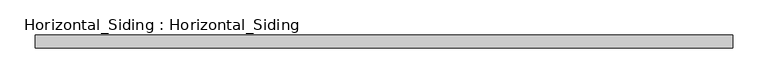
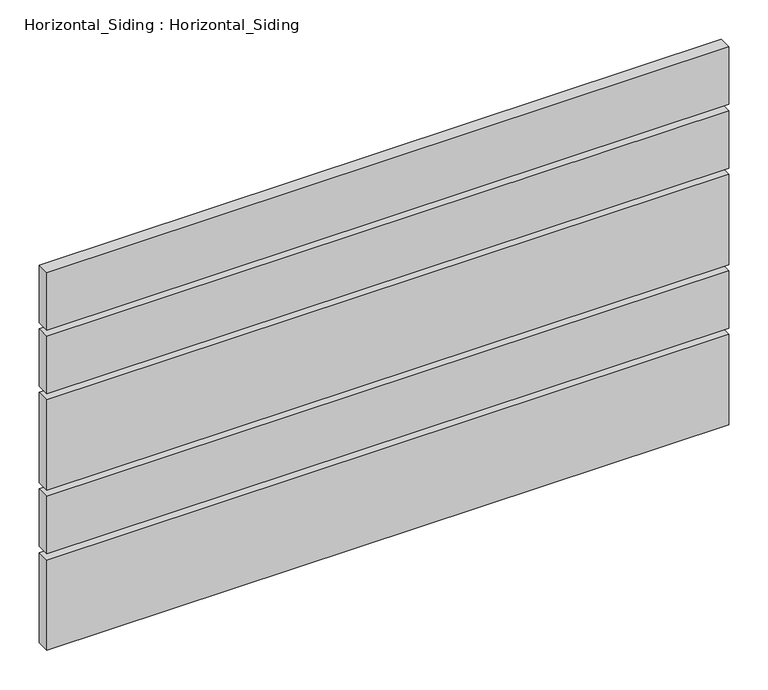
"""IFC4 building model written with IfcOpenShell, lengths in millimetres: plate geometry, Horizontal_Siding : Horizontal_Siding."""

from ifc_helpers import new_model, si_unit, frame, origin, place, context, project, spatial, polyline, outline, extrude, source, transform, mapped, element, save


def horizontal_siding_horizontal_siding_58939094(model_context):
    return source(origin(), model_context, "Body", "SweptSolid", [
        extrude(outline(polyline([(498.475, -19.05), (-498.475, -19.05), (-498.475, 0.0), (498.475, 0.0), (498.475, -19.05)])), frame((0.0, 0.0, 9.525), z_axis=(0.0, 0.0, 1.0), x_axis=(1.0, 0.0, 0.0)), (0.0, 0.0, 1.0), 139.7),
        extrude(outline(polyline([(498.475, -19.05), (-498.475, -19.05), (-498.475, 0.0), (498.475, 0.0), (498.475, -19.05)])), frame((0.0, 0.0, 158.75), z_axis=(0.0, 0.0, 1.0), x_axis=(1.0, 0.0, 0.0)), (0.0, 0.0, 1.0), 88.9),
        extrude(outline(polyline([(498.475, -19.05), (-498.475, -19.05), (-498.475, 0.0), (498.475, 0.0), (498.475, -19.05)])), frame((0.0, 0.0, 257.175), z_axis=(0.0, 0.0, 1.0), x_axis=(1.0, 0.0, 0.0)), (0.0, 0.0, 1.0), 139.7),
        extrude(outline(polyline([(498.475, -19.05), (-498.475, -19.05), (-498.475, 0.0), (498.475, 0.0), (498.475, -19.05)])), frame((0.0, 0.0, 406.4), z_axis=(0.0, 0.0, 1.0), x_axis=(1.0, 0.0, 0.0)), (0.0, 0.0, 1.0), 88.9),
        extrude(outline(polyline([(498.475, -19.05), (-498.475, -19.05), (-498.475, 0.0), (498.475, 0.0), (498.475, -19.05)])), frame((0.0, 0.0, 504.825), z_axis=(0.0, 0.0, 1.0), x_axis=(1.0, 0.0, 0.0)), (0.0, 0.0, 1.0), 88.9),
    ])


if __name__ == "__main__":
    model = new_model("IFC4")
    model_context = context("Model", 3, world=origin())
    ifc_project = project(units=[si_unit("LENGTHUNIT", "METRE", prefix="MILLI")], contexts=[model_context])
    site = spatial("IfcSite", under=ifc_project)
    building = spatial("IfcBuilding", under=site)
    placement = place(None, origin())
    horizontal_siding_horizontal_siding_shape = horizontal_siding_horizontal_siding_58939094(model_context)
    element("IfcPlate", 1, ObjectType="Horizontal_Siding : Horizontal_Siding", at=placement, inside=building, context=model_context, shape_type="MappedRepresentation", body=[
        mapped(horizontal_siding_horizontal_siding_shape, transform((0.0, 0.0, 0.0), x_axis=(1.0, 0.0, 0.0), y_axis=(0.0, 1.0, 0.0), z_axis=(0.0, 0.0, 1.0))),
    ])
    save(model, "model.ifc")

# Revit data of these elements
# Type "Horizontal_Siding : Horizontal_Siding"
#   Type Mark = "OUT"
#   Analytic Construction = "<None>"
#   extend = 0' - 2 3/4"
#   Width_2 = 0' - 3 1/2"
#   Width_1 = 0' - 5 1/2"
#   Gap = 0' - 0 3/8"
#   Plank Material = SLOTTED WOOD FENCE (THERMALLY MODIFIED WOOD: ARBOR WOOD)\n(EXTERIOR STAIN : PENOFIN VERDE EXT. STAIN - COLOR: CEDAR)
# Element 1 (IfcPlate, "Horizontal_Siding : Horizontal_Siding")
#   Materials on its faces: "SLOTTED WOOD FENCE (THERMALLY MODIFIED WOOD: ARBOR WOOD)\n(EXTERIOR STAIN : PENOFIN VERDE EXT. STAIN - COLOR: CEDAR)"
# Materials
#   "SLOTTED WOOD FENCE (THERMALLY MODIFIED WOOD: ARBOR WOOD)\n(EXTERIOR STAIN : PENOFIN VERDE EXT. STAIN - COLOR: CEDAR)": class "Wood", colour RGB 164 134 123, transparency 0, Description = "Pinus Echinata", Cost = 0
